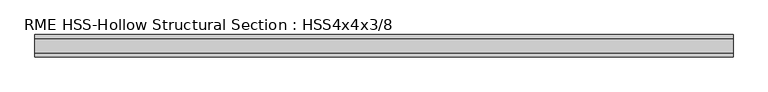
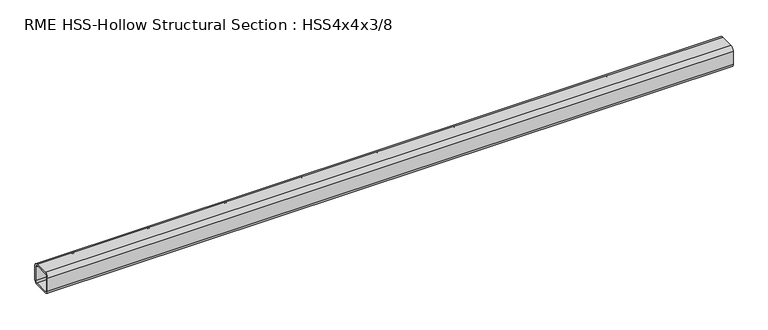
"""IFC4 building model written with IfcOpenShell, lengths in millimetres: member geometry, RME HSS-Hollow Structural Section : HSS4x4x3/8."""

from ifc_helpers import new_model, si_unit, point, frame, frame_2d, origin, place, context, project, spatial, polyline, circle_curve, trimmed, segment, composite_curve, outline, extrude, source, transform, mapped, element, save


def rme_hss_hollow_structural_section_hss4x4x3_8_c599a284(model_context):
    return source(origin(), model_context, "Body", "SweptSolid", [
        extrude(outline(composite_curve([segment(polyline([(50.8, 33.0708), (50.8, -33.0708)]), True, "CONTINUOUS"), segment(trimmed(circle_curve(frame_2d((33.0708, -33.0708)), 17.7292), [point((50.8, -33.0708))], [point((33.0708, -50.8))], False, "CARTESIAN"), True, "CONTINUOUS"), segment(polyline([(33.0708, -50.8), (-33.0708, -50.8)]), True, "CONTINUOUS"), segment(trimmed(circle_curve(frame_2d((-33.0708, -33.0708)), 17.7292), [point((-33.0708, -50.8))], [point((-50.8, -33.0708))], False, "CARTESIAN"), True, "CONTINUOUS"), segment(polyline([(-50.8, -33.0708), (-50.8, 33.0708)]), True, "CONTINUOUS"), segment(trimmed(circle_curve(frame_2d((-33.0708, 33.0708)), 17.7292), [point((-50.8, 33.0708))], [point((-33.0708, 50.8))], False, "CARTESIAN"), True, "CONTINUOUS"), segment(polyline([(-33.0708, 50.8), (33.0708, 50.8)]), True, "CONTINUOUS"), segment(trimmed(circle_curve(frame_2d((33.0708, 33.0708)), 17.7292), [point((33.0708, 50.8))], [point((50.8, 33.0708))], False, "CARTESIAN"), True, "CONTINUOUS")], self_intersect=False), holes=[composite_curve([segment(trimmed(circle_curve(frame_2d((-33.0708, 33.0708)), 8.8646), [point((-33.0708, 41.9354))], [point((-41.9354, 33.0708))], True, "CARTESIAN"), True, "CONTINUOUS"), segment(polyline([(-41.9354, 33.0708), (-41.9354, -33.0708)]), True, "CONTINUOUS"), segment(trimmed(circle_curve(frame_2d((-33.0708, -33.0708)), 8.8646), [point((-41.9354, -33.0708))], [point((-33.0708, -41.9354))], True, "CARTESIAN"), True, "CONTINUOUS"), segment(polyline([(-33.0708, -41.9354), (33.0708, -41.9354)]), True, "CONTINUOUS"), segment(trimmed(circle_curve(frame_2d((33.0708, -33.0708)), 8.8646), [point((33.0708, -41.9354))], [point((41.9354, -33.0708))], True, "CARTESIAN"), True, "CONTINUOUS"), segment(polyline([(41.9354, -33.0708), (41.9354, 33.0708)]), True, "CONTINUOUS"), segment(trimmed(circle_curve(frame_2d((33.0708, 33.0708)), 8.8646), [point((41.9354, 33.0708))], [point((33.0708, 41.9354))], True, "CARTESIAN"), True, "CONTINUOUS"), segment(polyline([(33.0708, 41.9354), (-33.0708, 41.9354)]), True, "CONTINUOUS")], self_intersect=False)]), frame((-1501.7244081, 0.0, 0.0), z_axis=(1.0, 0.0, 0.0), x_axis=(0.0, 1.0, 0.0)), (0.0, 0.0, 1.0), 3196.9810285),
    ])


if __name__ == "__main__":
    model = new_model("IFC4")
    model_context = context("Model", 3, world=origin())
    ifc_project = project(units=[si_unit("LENGTHUNIT", "METRE", prefix="MILLI")], contexts=[model_context])
    site = spatial("IfcSite", under=ifc_project)
    building = spatial("IfcBuilding", under=site)
    placement = place(None, origin())
    rme_hss_hollow_structural_section_hss4x4x3_8_shape = rme_hss_hollow_structural_section_hss4x4x3_8_c599a284(model_context)
    element("IfcMember", 1, ObjectType="RME HSS-Hollow Structural Section : HSS4x4x3/8", at=placement, inside=building, context=model_context, shape_type="MappedRepresentation", body=[
        mapped(rme_hss_hollow_structural_section_hss4x4x3_8_shape, transform((0.0, 0.0, 0.0), x_axis=(1.0, 0.0, 0.0), y_axis=(0.0, 1.0, 0.0), z_axis=(0.0, 0.0, 1.0))),
    ])
    save(model, "model.ifc")

# Revit data of these elements
# Type "RME HSS-Hollow Structural Section : HSS4x4x3/8"
#   Nominal Size = "HSS6x4"
#   Assembly Code = "B10"
#   Shape = "Square"
#   W = 17.2
#   Start Extension Calculation [instance default] = 10' - 0"
#   Start Extension [instance default] = -0' - 0 1/2"
#   End Extension Calculation [instance default] = 10' - 0"
#   End Extension [instance default] = -0' - 0 1/2"
#   Ht = 0' - 4"
#   Length [instance default] = 5' - 0"
#   b = 0' - 4"
#   kr = 0' - 0.698"
#   t = 0' - 0.349"
#   A = 0.0331944 SF
#   Structural Material [instance default] = Metal - Steel - ASTM A500 - Grade B - Rectangular and Square
# Element 1 (IfcMember, "RME HSS-Hollow Structural Section : HSS4x4x3/8")
#   End Extension Calculation = 9' - 7.24239"
#   End Extension = -0' - 5.25761"
#   Length = 11' - 11"
#   Structural Material = Metal - Steel - ASTM A992
#   Materials on its faces: "Metal - Steel - ASTM A992"
# Materials
#   "Metal - Steel - ASTM A500 - Grade B - Rectangular and Square": class "Metal", colour RGB 255 128 0, transparency 0
#   "Metal - Steel - ASTM A992": class "Metal", colour RGB 255 128 0, transparency 0
